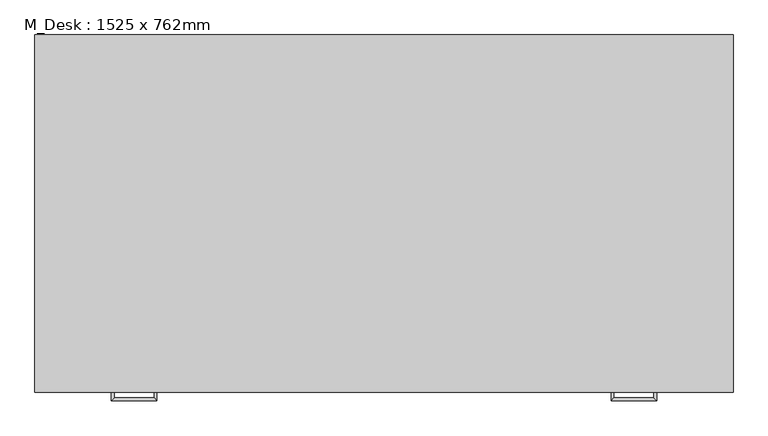
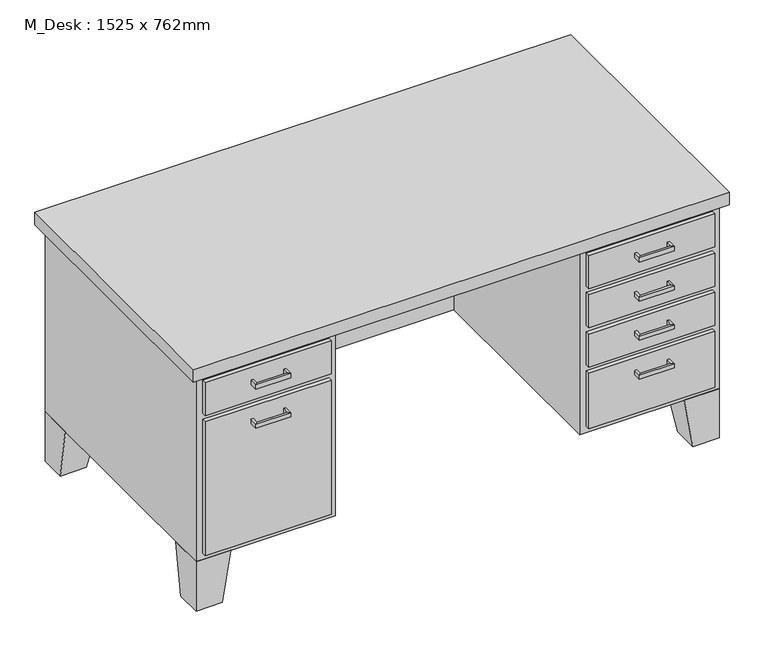
"""IFC4 building model written with IfcOpenShell, lengths in millimetres: furniture geometry, M_Desk : 1525 x 762mm."""

from ifc_helpers import new_model, si_unit, frame, origin, place, context, project, spatial, polyline, outline, extrude, faceted_brep, source, transform, mapped, element, save


def m_desk_1525_x_762mm_8f660baf(model_context):
    return source(origin(), model_context, "Body", "SolidModel", [
        extrude(outline(polyline([(18.55, 0.0), (386.85, 0.0), (386.85, -12.7), (18.55, -12.7), (18.55, 0.0)])), frame((0.0, 0.0, 603.25), z_axis=(0.0, 0.0, 1.0), x_axis=(1.0, 0.0, 0.0)), (0.0, 0.0, 1.0), 101.6),
        extrude(outline(polyline([(18.55, 0.0), (386.85, 0.0), (386.85, -12.7), (18.55, -12.7), (18.55, 0.0)])), frame((0.0, 0.0, 171.05), z_axis=(0.0, 0.0, 1.0), x_axis=(1.0, 0.0, 0.0)), (0.0, 0.0, 1.0), 413.15),
        extrude(outline(polyline([(1137.15, 0.0), (1505.45, 0.0), (1505.45, -12.7), (1137.15, -12.7), (1137.15, 0.0)])), frame((0.0, 0.0, 602.85), z_axis=(0.0, 0.0, 1.0), x_axis=(1.0, 0.0, 0.0)), (0.0, 0.0, 1.0), 102.0),
        extrude(outline(polyline([(1137.15, 0.0), (1505.45, 0.0), (1505.45, -12.7), (1137.15, -12.7), (1137.15, 0.0)])), frame((0.0, 0.0, 171.05), z_axis=(0.0, 0.0, 1.0), x_axis=(1.0, 0.0, 0.0)), (0.0, 0.0, 1.0), 171.45),
        extrude(outline(polyline([(1137.15, 0.0), (1505.45, 0.0), (1505.45, -12.7), (1137.15, -12.7), (1137.15, 0.0)])), frame((0.0, 0.0, 482.2), z_axis=(0.0, 0.0, 1.0), x_axis=(1.0, 0.0, 0.0)), (0.0, 0.0, 1.0), 101.6),
        extrude(outline(polyline([(1137.15, 0.0), (1505.45, 0.0), (1505.45, -12.7), (1137.15, -12.7), (1137.15, 0.0)])), frame((0.0, 0.0, 361.55), z_axis=(0.0, 0.0, 1.0), x_axis=(1.0, 0.0, 0.0)), (0.0, 0.0, 1.0), 101.6),
        faceted_brep([(101.1, 0.0, 152.0), (101.1, 101.6, 152.0), (-0.5, 101.6, 152.0), (-0.5, 0.0, 152.0), (75.7, 0.0, 0.0), (-0.5, 0.0, 0.0), (-0.5, 76.2, 0.0), (75.7, 76.2, 0.0)], [[[0, 1, 2, 3]], [[4, 5, 6, 7]], [[4, 7, 1, 0]], [[7, 6, 2, 1]], [[6, 5, 3, 2]], [[5, 4, 0, 3]]]),
        faceted_brep([(101.1, 762.0, 152.0), (-0.5, 762.0, 152.0), (-0.5, 660.4, 152.0), (101.1, 660.4, 152.0), (75.7, 762.0, 0.0), (75.7, 685.8, 0.0), (-0.5, 685.8, 0.0), (-0.5, 762.0, 0.0)], [[[0, 1, 2, 3]], [[4, 5, 6, 7]], [[4, 7, 1, 0]], [[7, 6, 2, 1]], [[6, 5, 3, 2]], [[5, 4, 0, 3]]]),
        faceted_brep([(1422.9, 762.0, 152.0), (1422.9, 660.4, 152.0), (1524.5, 660.4, 152.0), (1524.5, 762.0, 152.0), (1448.3, 762.0, 0.0), (1524.5, 762.0, 0.0), (1524.5, 685.8, 0.0), (1448.3, 685.8, 0.0)], [[[0, 1, 2, 3]], [[4, 5, 6, 7]], [[4, 7, 1, 0]], [[7, 6, 2, 1]], [[6, 5, 3, 2]], [[5, 4, 0, 3]]]),
        faceted_brep([(1422.9, 0.0, 152.0), (1524.5, 0.0, 152.0), (1524.5, 101.6, 152.0), (1422.9, 101.6, 152.0), (1448.3, 0.0, 0.0), (1448.3, 76.2, 0.0), (1524.5, 76.2, 0.0), (1524.5, 0.0, 0.0)], [[[0, 1, 2, 3]], [[4, 5, 6, 7]], [[4, 7, 1, 0]], [[7, 6, 2, 1]], [[6, 5, 3, 2]], [[5, 4, 0, 3]]]),
        extrude(outline(polyline([(-19.55, -19.05), (-19.55, 781.05), (1543.55, 781.05), (1543.55, -19.05), (-19.55, -19.05)])), frame((0.0, 0.0, 723.9), z_axis=(0.0, 0.0, 1.0), x_axis=(1.0, 0.0, 0.0)), (0.0, 0.0, 1.0), 38.1),
        extrude(outline(polyline([(1118.1, 0.0), (1118.1, 635.0), (405.9, 635.0), (405.9, 0.0), (-0.5, 0.0), (-0.5, 762.0), (1524.5, 762.0), (1524.5, 0.0), (1118.1, 0.0)])), frame((0.0, 0.0, 152.0), z_axis=(0.0, 0.0, 1.0), x_axis=(1.0, 0.0, 0.0)), (0.0, 0.0, 1.0), 571.9),
        faceted_brep([(158.25, -12.7, 546.1), (158.25, -12.7, 533.4), (151.9, -12.7, 533.4), (151.9, -12.7, 546.1), (158.25, -31.75, 546.1), (158.25, -31.75, 533.4), (151.9, -38.1, 533.4), (151.9, -38.1, 546.1), (247.15, -31.75, 546.1), (247.15, -31.75, 533.4), (253.5, -38.1, 533.4), (253.5, -38.1, 546.1), (247.15, -12.7, 546.1), (253.5, -12.7, 546.1), (253.5, -12.7, 533.4), (247.15, -12.7, 533.4)], [[[0, 1, 2, 3]], [[1, 0, 4, 5]], [[2, 1, 5, 6]], [[3, 2, 6, 7]], [[0, 3, 7, 4]], [[5, 4, 8, 9]], [[6, 5, 9, 10]], [[7, 6, 10, 11]], [[4, 7, 11, 8]], [[12, 13, 14, 15]], [[9, 8, 12, 15]], [[10, 9, 15, 14]], [[11, 10, 14, 13]], [[8, 11, 13, 12]]]),
        faceted_brep([(158.25, -12.7, 666.75), (158.25, -12.7, 654.05), (151.9, -12.7, 654.05), (151.9, -12.7, 666.75), (158.25, -31.75, 666.75), (158.25, -31.75, 654.05), (151.9, -38.1, 654.05), (151.9, -38.1, 666.75), (247.15, -31.75, 666.75), (247.15, -31.75, 654.05), (253.5, -38.1, 654.05), (253.5, -38.1, 666.75), (247.15, -12.7, 666.75), (253.5, -12.7, 666.75), (253.5, -12.7, 654.05), (247.15, -12.7, 654.05)], [[[0, 1, 2, 3]], [[1, 0, 4, 5]], [[2, 1, 5, 6]], [[3, 2, 6, 7]], [[0, 3, 7, 4]], [[5, 4, 8, 9]], [[6, 5, 9, 10]], [[7, 6, 10, 11]], [[4, 7, 11, 8]], [[12, 13, 14, 15]], [[9, 8, 12, 15]], [[10, 9, 15, 14]], [[11, 10, 14, 13]], [[8, 11, 13, 12]]]),
        faceted_brep([(1365.75, -12.7, 304.8), (1372.1, -12.7, 304.8), (1372.1, -12.7, 292.1), (1365.75, -12.7, 292.1), (1365.75, -31.75, 304.8), (1372.1, -38.1, 304.8), (1372.1, -38.1, 292.1), (1365.75, -31.75, 292.1), (1276.85, -31.75, 304.8), (1270.5, -38.1, 304.8), (1270.5, -38.1, 292.1), (1276.85, -31.75, 292.1), (1276.85, -12.7, 304.8), (1276.85, -12.7, 292.1), (1270.5, -12.7, 292.1), (1270.5, -12.7, 304.8)], [[[0, 1, 2, 3]], [[1, 0, 4, 5]], [[2, 1, 5, 6]], [[3, 2, 6, 7]], [[0, 3, 7, 4]], [[5, 4, 8, 9]], [[6, 5, 9, 10]], [[7, 6, 10, 11]], [[4, 7, 11, 8]], [[12, 13, 14, 15]], [[9, 8, 12, 15]], [[10, 9, 15, 14]], [[11, 10, 14, 13]], [[8, 11, 13, 12]]]),
        faceted_brep([(1365.75, -12.7, 425.45), (1372.1, -12.7, 425.45), (1372.1, -12.7, 412.75), (1365.75, -12.7, 412.75), (1365.75, -31.75, 425.45), (1372.1, -38.1, 425.45), (1372.1, -38.1, 412.75), (1365.75, -31.75, 412.75), (1276.85, -31.75, 425.45), (1270.5, -38.1, 425.45), (1270.5, -38.1, 412.75), (1276.85, -31.75, 412.75), (1276.85, -12.7, 425.45), (1276.85, -12.7, 412.75), (1270.5, -12.7, 412.75), (1270.5, -12.7, 425.45)], [[[0, 1, 2, 3]], [[1, 0, 4, 5]], [[2, 1, 5, 6]], [[3, 2, 6, 7]], [[0, 3, 7, 4]], [[5, 4, 8, 9]], [[6, 5, 9, 10]], [[7, 6, 10, 11]], [[4, 7, 11, 8]], [[12, 13, 14, 15]], [[9, 8, 12, 15]], [[10, 9, 15, 14]], [[11, 10, 14, 13]], [[8, 11, 13, 12]]]),
        faceted_brep([(1365.75, -12.7, 546.1), (1372.1, -12.7, 546.1), (1372.1, -12.7, 533.4), (1365.75, -12.7, 533.4), (1365.75, -31.75, 546.1), (1372.1, -38.1, 546.1), (1372.1, -38.1, 533.4), (1365.75, -31.75, 533.4), (1276.85, -31.75, 546.1), (1270.5, -38.1, 546.1), (1270.5, -38.1, 533.4), (1276.85, -31.75, 533.4), (1276.85, -12.7, 546.1), (1276.85, -12.7, 533.4), (1270.5, -12.7, 533.4), (1270.5, -12.7, 546.1)], [[[0, 1, 2, 3]], [[1, 0, 4, 5]], [[2, 1, 5, 6]], [[3, 2, 6, 7]], [[0, 3, 7, 4]], [[5, 4, 8, 9]], [[6, 5, 9, 10]], [[7, 6, 10, 11]], [[4, 7, 11, 8]], [[12, 13, 14, 15]], [[9, 8, 12, 15]], [[10, 9, 15, 14]], [[11, 10, 14, 13]], [[8, 11, 13, 12]]]),
        faceted_brep([(1365.75, -12.7, 666.75), (1372.1, -12.7, 666.75), (1372.1, -12.7, 654.05), (1365.75, -12.7, 654.05), (1365.75, -31.75, 666.75), (1372.1, -38.1, 666.75), (1372.1, -38.1, 654.05), (1365.75, -31.75, 654.05), (1276.85, -31.75, 666.75), (1270.5, -38.1, 666.75), (1270.5, -38.1, 654.05), (1276.85, -31.75, 654.05), (1276.85, -12.7, 666.75), (1276.85, -12.7, 654.05), (1270.5, -12.7, 654.05), (1270.5, -12.7, 666.75)], [[[0, 1, 2, 3]], [[1, 0, 4, 5]], [[2, 1, 5, 6]], [[3, 2, 6, 7]], [[0, 3, 7, 4]], [[5, 4, 8, 9]], [[6, 5, 9, 10]], [[7, 6, 10, 11]], [[4, 7, 11, 8]], [[12, 13, 14, 15]], [[9, 8, 12, 15]], [[10, 9, 15, 14]], [[11, 10, 14, 13]], [[8, 11, 13, 12]]]),
    ])


if __name__ == "__main__":
    model = new_model("IFC4")
    model_context = context("Model", 3, world=origin())
    ifc_project = project(units=[si_unit("LENGTHUNIT", "METRE", prefix="MILLI")], contexts=[model_context])
    site = spatial("IfcSite", under=ifc_project)
    building = spatial("IfcBuilding", under=site)
    placement = place(None, origin())
    m_desk_1525_x_762mm_shape = m_desk_1525_x_762mm_8f660baf(model_context)
    element("IfcFurniture", 1, ObjectType="M_Desk : 1525 x 762mm", at=placement, inside=building, context=model_context, shape_type="MappedRepresentation", body=[
        mapped(m_desk_1525_x_762mm_shape, transform((0.0, 0.0, 0.0), x_axis=(1.0, 0.0, 0.0), y_axis=(0.0, 1.0, 0.0), z_axis=(0.0, 0.0, 1.0))),
    ])
    save(model, "model.ifc")

# Revit data of these elements
# Type "M_Desk : 1525 x 762mm"
#   Depth = 0.762 m
#   Height = 0.762 m
#   Leg Height = 0.152 m
#   Width = 1.525 m
#   Body Material = Laminate, Ivory, Matte
#   Handle/Leg Material = Steel, Chrome Plated
#   Top Material = Cherry
#   Assembly Code = ""
# Element 1 (IfcFurniture, "M_Desk : 1525 x 762mm")
#   Materials on its faces: "Steel, Chrome Plated", "Laminate, Ivory, Matte", "Cherry"
# Materials
#   "Laminate, Ivory, Matte": class "Plastic", colour RGB 247 247 229, transparency 0, Description = "Plastic Laminate - Ivory, Matte", Cost = 0
#   "Steel, Chrome Plated": class "Metal", colour RGB 244 244 244, transparency 0, Description = "Chromiuim plated steel", Cost = 0
#   "Cherry": class "Wood", colour RGB 154 107 61, transparency 0, Description = "Prunus Serotina", Cost = 0
